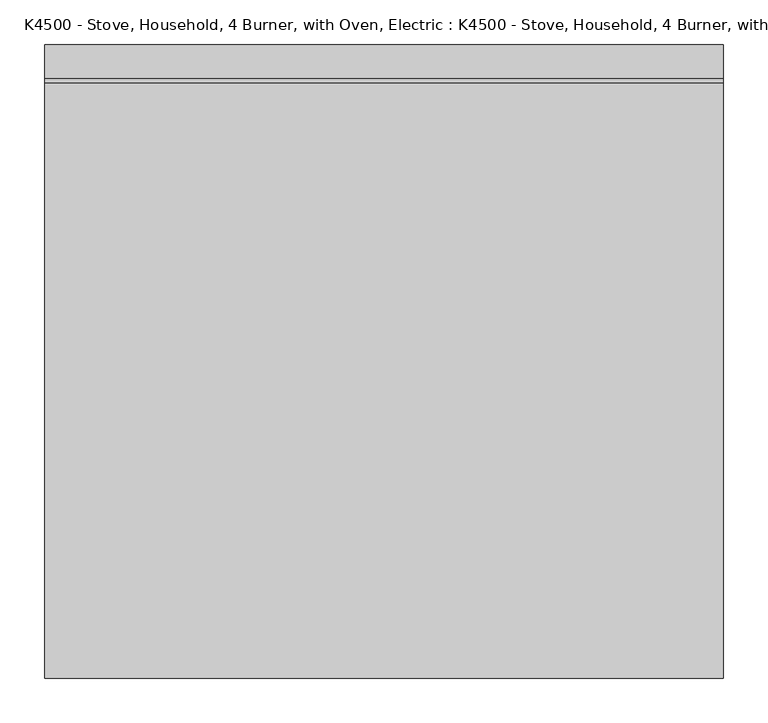
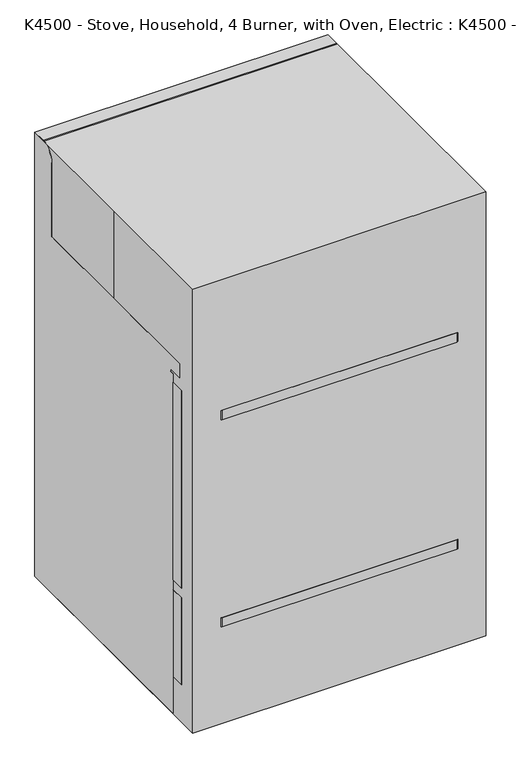
"""IFC4 building model written with IfcOpenShell, lengths in millimetres: proxy geometry, K4500 - Stove, Household, 4 Burner, with Oven, Electric : K4500 - Stove, Household, 4 Burner, with Oven, Electric."""

from ifc_helpers import new_model, si_unit, point, frame, frame_2d, origin, origin_with_axes, place, context, project, spatial, polyline, circle_curve, trimmed, segment, composite_curve, outline, extrude, source, transform, mapped, element, save


def k4500_stove_household_4_burner_with_oven_electric_k4500_e1e5008a(model_context):
    return source(origin(), model_context, "Body", "SweptSolid", [
        extrude(outline(composite_curve([segment(trimmed(circle_curve(frame_2d((-200.0809431, 110.6842635)), 127.0), [point((-200.0809431, -16.3157365))], [point((-200.0809431, 237.6842635))], False, "CARTESIAN"), True, "CONTINUOUS"), segment(trimmed(circle_curve(frame_2d((-200.0809431, 110.6842635)), 127.0), [point((-200.0809431, 237.6842635))], [point((-200.0809431, -16.3157365))], False, "CARTESIAN"), True, "CONTINUOUS")], self_intersect=False)), frame((0.0, 0.0, 977.9), z_axis=(0.0, 0.0, 1.0), x_axis=(1.0, 0.0, 0.0)), (0.0, 0.0, 1.0), 1.6611193),
        extrude(outline(composite_curve([segment(trimmed(circle_curve(frame_2d((-201.1618656, -149.6657365)), 101.6), [point((-201.1618656, -251.2657365))], [point((-201.1618656, -48.0657365))], False, "CARTESIAN"), True, "CONTINUOUS"), segment(trimmed(circle_curve(frame_2d((-201.1618656, -149.6657365)), 101.6), [point((-201.1618656, -48.0657365))], [point((-201.1618656, -251.2657365))], False, "CARTESIAN"), True, "CONTINUOUS")], self_intersect=False)), frame((0.0, 0.0, 977.9), z_axis=(0.0, 0.0, 1.0), x_axis=(1.0, 0.0, 0.0)), (0.0, 0.0, 1.0), 1.6611193),
        extrude(outline(composite_curve([segment(trimmed(circle_curve(frame_2d((179.8381344, -130.6157365)), 127.0), [point((179.8381344, -257.6157365))], [point((179.8381344, -3.6157365))], False, "CARTESIAN"), True, "CONTINUOUS"), segment(trimmed(circle_curve(frame_2d((179.8381344, -130.6157365)), 127.0), [point((179.8381344, -3.6157365))], [point((179.8381344, -257.6157365))], False, "CARTESIAN"), True, "CONTINUOUS")], self_intersect=False)), frame((0.0, 0.0, 977.9), z_axis=(0.0, 0.0, 1.0), x_axis=(1.0, 0.0, 0.0)), (0.0, 0.0, 1.0), 1.6611193),
        extrude(outline(composite_curve([segment(trimmed(circle_curve(frame_2d((179.8381344, 129.7342635)), 101.6), [point((179.8381344, 28.1342635))], [point((179.8381344, 231.3342635))], False, "CARTESIAN"), True, "CONTINUOUS"), segment(trimmed(circle_curve(frame_2d((179.8381344, 129.7342635)), 101.6), [point((179.8381344, 231.3342635))], [point((179.8381344, 28.1342635))], False, "CARTESIAN"), True, "CONTINUOUS")], self_intersect=False)), frame((0.0, 0.0, 977.9), z_axis=(0.0, 0.0, 1.0), x_axis=(1.0, 0.0, 0.0)), (0.0, 0.0, 1.0), 1.6611193),
        extrude(outline(composite_curve([segment(trimmed(circle_curve(frame_2d((1096.7029969, -242.3422997)), 25.4), [point((1096.7029969, -267.7422997))], [point((1096.7029969, -216.9422997))], False, "CARTESIAN"), True, "CONTINUOUS"), segment(trimmed(circle_curve(frame_2d((1096.7029969, -242.3422997)), 25.4), [point((1096.7029969, -216.9422997))], [point((1096.7029969, -267.7422997))], False, "CARTESIAN"), True, "CONTINUOUS")], self_intersect=False)), frame((0.0, 266.7, 0.0), z_axis=(0.0, 1.0, 0.0), x_axis=(0.0, 0.0, 1.0)), (0.0, 0.0, 1.0), 12.7),
        extrude(outline(composite_curve([segment(trimmed(circle_curve(frame_2d((1096.7029969, -321.7172997)), 25.4), [point((1096.7029969, -347.1172997))], [point((1096.7029969, -296.3172997))], False, "CARTESIAN"), True, "CONTINUOUS"), segment(trimmed(circle_curve(frame_2d((1096.7029969, -321.7172997)), 25.4), [point((1096.7029969, -296.3172997))], [point((1096.7029969, -347.1172997))], False, "CARTESIAN"), True, "CONTINUOUS")], self_intersect=False)), frame((0.0, 266.7, 0.0), z_axis=(0.0, 1.0, 0.0), x_axis=(0.0, 0.0, 1.0)), (0.0, 0.0, 1.0), 12.7),
        extrude(outline(polyline([(101.6, 273.05), (-101.6, 273.05), (-101.6, 279.4), (101.6, 279.4), (101.6, 273.05)])), frame((0.0, 0.0, 1057.3840399), z_axis=(0.0, 0.0, 1.0), x_axis=(1.0, 0.0, 0.0)), (0.0, 0.0, 1.0), 80.0902197),
        extrude(outline(composite_curve([segment(trimmed(circle_curve(frame_2d((1096.7029969, 162.9672997)), 25.4), [point((1096.7029969, 188.3672997))], [point((1096.7029969, 137.5672997))], False, "CARTESIAN"), True, "CONTINUOUS"), segment(trimmed(circle_curve(frame_2d((1096.7029969, 162.9672997)), 25.4), [point((1096.7029969, 137.5672997))], [point((1096.7029969, 188.3672997))], False, "CARTESIAN"), True, "CONTINUOUS")], self_intersect=False)), frame((0.0, 266.7, 0.0), z_axis=(0.0, 1.0, 0.0), x_axis=(0.0, 0.0, 1.0)), (0.0, 0.0, 1.0), 12.7),
        extrude(outline(composite_curve([segment(trimmed(circle_curve(frame_2d((1096.7029969, 242.3422997)), 25.4), [point((1096.7029969, 267.7422997))], [point((1096.7029969, 216.9422997))], False, "CARTESIAN"), True, "CONTINUOUS"), segment(trimmed(circle_curve(frame_2d((1096.7029969, 242.3422997)), 25.4), [point((1096.7029969, 216.9422997))], [point((1096.7029969, 267.7422997))], False, "CARTESIAN"), True, "CONTINUOUS")], self_intersect=False)), frame((0.0, 266.7, 0.0), z_axis=(0.0, 1.0, 0.0), x_axis=(0.0, 0.0, 1.0)), (0.0, 0.0, 1.0), 12.7),
        extrude(outline(composite_curve([segment(trimmed(circle_curve(frame_2d((1096.7029969, 321.7172997)), 25.4), [point((1096.7029969, 347.1172997))], [point((1096.7029969, 296.3172997))], False, "CARTESIAN"), True, "CONTINUOUS"), segment(trimmed(circle_curve(frame_2d((1096.7029969, 321.7172997)), 25.4), [point((1096.7029969, 296.3172997))], [point((1096.7029969, 347.1172997))], False, "CARTESIAN"), True, "CONTINUOUS")], self_intersect=False)), frame((0.0, 266.7, 0.0), z_axis=(0.0, 1.0, 0.0), x_axis=(0.0, 0.0, 1.0)), (0.0, 0.0, 1.0), 12.7),
        extrude(outline(composite_curve([segment(polyline([(-323.8497807, -304.7959776), (-317.4997807, -304.7959776), (-317.4997807, -336.5459776)]), True, "CONTINUOUS"), segment(trimmed(circle_curve(frame_2d((-304.7997807, -336.5459776)), 12.7), [point((-317.4997807, -336.5459776))], [point((-304.7997807, -349.2459776))], True, "CARTESIAN"), True, "CONTINUOUS"), segment(polyline([(-304.7997807, -349.2459776), (304.8002193, -349.2459776)]), True, "CONTINUOUS"), segment(trimmed(circle_curve(frame_2d((304.8002193, -336.5459776)), 12.7), [point((304.8002193, -349.2459776))], [point((317.5002193, -336.5459776))], True, "CARTESIAN"), True, "CONTINUOUS"), segment(polyline([(317.5002193, -336.5459776), (317.5002193, -304.7959776), (323.8502193, -304.7959776), (323.8502193, -336.5459776)]), True, "CONTINUOUS"), segment(trimmed(circle_curve(frame_2d((304.8002193, -336.5459776)), 19.05), [point((323.8502193, -336.5459776))], [point((304.8002193, -355.5959776))], False, "CARTESIAN"), True, "CONTINUOUS"), segment(polyline([(304.8002193, -355.5959776), (-304.7997807, -355.5959776)]), True, "CONTINUOUS"), segment(trimmed(circle_curve(frame_2d((-304.7997807, -336.5459776)), 19.05), [point((-304.7997807, -355.5959776))], [point((-323.8497807, -336.5459776))], False, "CARTESIAN"), True, "CONTINUOUS"), segment(polyline([(-323.8497807, -336.5459776), (-323.8497807, -304.7959776)]), True, "CONTINUOUS")], self_intersect=False)), frame((0.0, 0.0, 833.8008351), z_axis=(0.0, 0.0, 1.0), x_axis=(1.0, 0.0, 0.0)), (0.0, 0.0, 1.0), 25.4),
        extrude(outline(polyline([(381.0, -304.8), (-381.0, -304.8), (-381.0, -266.7), (381.0, -266.7), (381.0, -304.8)])), frame((0.0, 0.0, 366.513372), z_axis=(0.0, 0.0, 1.0), x_axis=(1.0, 0.0, 0.0)), (0.0, 0.0, 1.0), 542.5081971),
        extrude(outline(composite_curve([segment(polyline([(-323.85, -304.8), (-317.5, -304.8), (-317.5, -336.55)]), True, "CONTINUOUS"), segment(trimmed(circle_curve(frame_2d((-304.8, -336.55)), 12.7), [point((-317.5, -336.55))], [point((-304.8, -349.25))], True, "CARTESIAN"), True, "CONTINUOUS"), segment(polyline([(-304.8, -349.25), (304.8, -349.25)]), True, "CONTINUOUS"), segment(trimmed(circle_curve(frame_2d((304.8, -336.55)), 12.7), [point((304.8, -349.25))], [point((317.5, -336.55))], True, "CARTESIAN"), True, "CONTINUOUS"), segment(polyline([(317.5, -336.55), (317.5, -304.8), (323.85, -304.8), (323.85, -336.55)]), True, "CONTINUOUS"), segment(trimmed(circle_curve(frame_2d((304.8, -336.55)), 19.05), [point((323.85, -336.55))], [point((304.8, -355.6))], False, "CARTESIAN"), True, "CONTINUOUS"), segment(polyline([(304.8, -355.6), (-304.8, -355.6)]), True, "CONTINUOUS"), segment(trimmed(circle_curve(frame_2d((-304.8, -336.55)), 19.05), [point((-304.8, -355.6))], [point((-323.85, -336.55))], False, "CARTESIAN"), True, "CONTINUOUS"), segment(polyline([(-323.85, -336.55), (-323.85, -304.8)]), True, "CONTINUOUS")], self_intersect=False)), frame((0.0, 0.0, 265.0511533), z_axis=(0.0, 0.0, 1.0), x_axis=(1.0, 0.0, 0.0)), (0.0, 0.0, 1.0), 25.4),
        extrude(outline(composite_curve([segment(polyline([(-266.7, 0.0), (-266.7, 933.45), (-255.696962, 933.45), (-255.696962, 939.8), (-296.1231495, 939.8), (-296.1231495, 977.9), (279.4, 977.9), (279.4, 1181.1)]), True, "CONTINUOUS"), segment(trimmed(circle_curve(frame_2d((317.5, 1181.1)), 38.1), [point((279.4, 1181.1))], [point((317.5, 1219.2))], False, "CARTESIAN"), True, "CONTINUOUS"), segment(polyline([(317.5, 1219.2), (355.6, 1219.2), (355.6, 0.0), (-266.7, 0.0)]), True, "CONTINUOUS")], self_intersect=False)), frame((-381.0, 0.0, 0.0), z_axis=(1.0, 0.0, 0.0), x_axis=(0.0, 1.0, 0.0)), (0.0, 0.0, 1.0), 762.0),
        extrude(outline(polyline([(381.0, -304.8), (-381.0, -304.8), (-381.0, -266.7), (381.0, -266.7), (381.0, -304.8)])), frame((0.0, 0.0, 101.5648187), z_axis=(0.0, 0.0, 1.0), x_axis=(1.0, 0.0, 0.0)), (0.0, 0.0, 1.0), 238.7070685),
        extrude(outline(polyline([(-381.0, 355.6), (381.0, 355.6), (381.0, -355.6), (-381.0, -355.6), (-381.0, 0.0), (-381.0, 355.6)])), origin_with_axes(), (0.0, 0.0, 1.0), 1219.2),
    ])


if __name__ == "__main__":
    model = new_model("IFC4")
    model_context = context("Model", 3, world=origin())
    ifc_project = project(units=[si_unit("LENGTHUNIT", "METRE", prefix="MILLI")], contexts=[model_context])
    site = spatial("IfcSite", under=ifc_project)
    building = spatial("IfcBuilding", under=site)
    placement = place(None, origin())
    k4500_stove_household_4_burner_with_oven_electric_k4500_shape = k4500_stove_household_4_burner_with_oven_electric_k4500_e1e5008a(model_context)
    element("IfcBuildingElementProxy", 1, Name="K4500 - Stove, Household, 4 Burner, with Oven, Electric : K4500 - Stove, Household, 4 Burner, with Oven, Electric", ObjectType="K4500 - Stove, Household, 4 Burner, with Oven, Electric : K4500 - Stove, Household, 4 Burner, with Oven, Electric", at=placement, inside=building, context=model_context, shape_type="MappedRepresentation", body=[
        mapped(k4500_stove_household_4_burner_with_oven_electric_k4500_shape, transform((0.0, 0.0, 0.0), x_axis=(1.0, 0.0, 0.0), y_axis=(0.0, 1.0, 0.0), z_axis=(0.0, 0.0, 1.0))),
    ])
    save(model, "model.ifc")

# Revit data of these elements
# Type "K4500 - Stove, Household, 4 Burner, with Oven, Electric : K4500 - Stove, Household, 4 Burner, with Oven, Electric"
#   Youtube clip = ""
#   Watts2 = "16628"
#   Watts1 = "14411"
#   Unit_Issue = "EA"
#   Uniclass 2.0 Description = ""
#   Uniclass 2.0 Code = ""
#   Uniclass 1.4 Description = ""
#   Uniclass 1.4 Code = ""
#   UTIL_6_Misc = "E"
#   UTIL_5_NonMedGas = "-"
#   UTIL_4_MiscGas = "-"
#   UTIL_3_MedGas = "-"
#   UTIL_2_Elec = "G"
#   UTIL_1_WaterDrain = "-"
#   UNSPSC Code = ""
#   Technical description = ""
#   Region South America = "None"
#   Region Oceania = "None"
#   Region North America = "US"
#   Region Middle East = "None"
#   Region Europe = "None"
#   Region Asia = "None"
#   Region Antarctica = "None"
#   Region Africa = "None"
#   QR code = "http://bimobject.com/seps2bim/product/K4500"
#   Product group = ""
#   Product family = ""
#   Product data url = "http://bimobject.com/seps2bim/product/K4500"
#   Product certification = ""
#   Product SKU = "K4500"
#   Product Guid = "64f65a7c-6c1d-4d24-9612-8fd2c08984c0"
#   OmniClass Description = ""
#   OmniClass Code = ""
#   Nomenclature = "Stove, Household, 4 Burner, with Oven, Electric"
#   NSN = "7310"
#   NBS Reference Description = ""
#   NBS Reference Code = ""
#   Material secondary = ""
#   Material main = ""
#   Manufacturer name = "SEPS2BIM"
#   Manufacturer country = "United States"
#   Location [instance default] = ""
#   JSN = "K4500"
#   Installation instructions = ""
#   IFC Classification = ""
#   Fund_Source_VA = "-"
#   Fund_Source_Navy = "-"
#   Fund_Source_Army = "-"
#   Fund_Source_AF = "-"
#   ELEC_Volts2 = "240"
#   ELEC_Volts1 = "208"
#   ELEC_Phase2 = "3"
#   ELEC_Phase1 = "3"
#   ELEC_HertzSwitch = "No"
#   ELEC_HertzDependent = "Yes"
#   ELEC_Hertz = "60"
#   ELEC_Amps2 = "40"
#   ELEC_Amps1 = "40"
#   EAN code = ""
#   DetailDescription = "Electric household range with four burner stove and oven.  Gas models are available.  This unit is used ni rehabilitation settings to teach daily living skills to patients."
#   Design country = "United States"
#   Description = "Electric household range with four burner stove and oven. Gas models are available. This unit is used in rehabilitation settings to teach daily living skills to patients."
#   Date of publishing = "2014-08-12"
#   COBIe Type Category = ""
#   CAT_VA = "A"
#   CAT_Navy = "A"
#   CAT_IHS = "-"
#   CAT_Army = "A"
#   CAT_AF = "A"
#   BTUperhour = "0"
#   BIMobject category = ""
#   Weight_IP = 190
#   Weight Net (Kg) = 0
#   Nominal width = 760
#   Nominal height = 1220
#   DIM_Width_IP = 2' - 6"
#   DIM_Height_IP = 4' - 0"
#   DIM_Depth_IP = 2' - 4"
#   Edition number = 1
#   Default Elevation = 0
# Element 1 (IfcBuildingElementProxy, "K4500 - Stove, Household, 4 Burner, with Oven, Electric : K4500 - Stove, Household, 4 Burner, with Oven, Electric")
#   Materials on its faces: "EquipSpace"
# Materials
#   "EquipSpace": class "Miscellaneous", colour RGB 221 217 195, transparency 0.5
